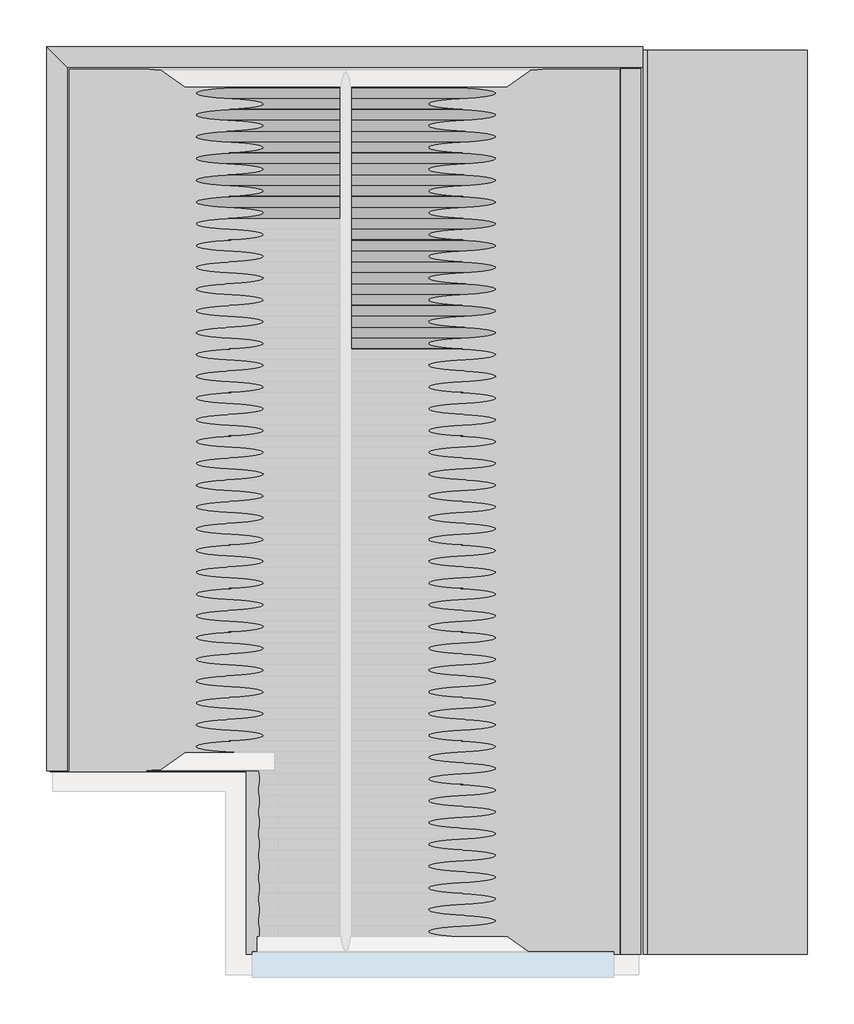
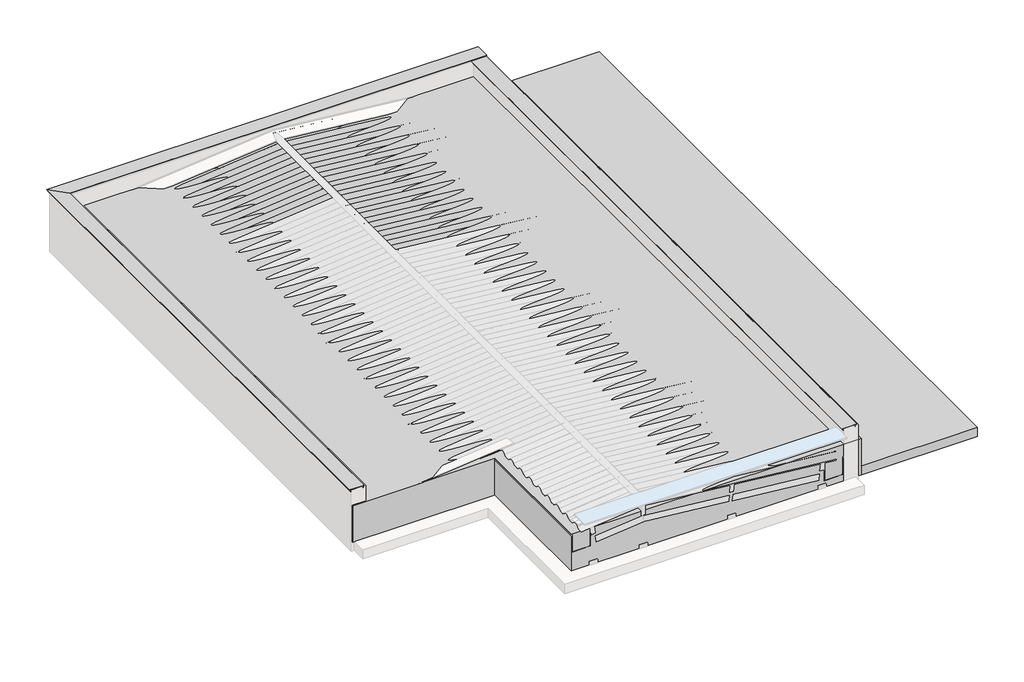
# One storey, part 4 of 4: 27 beams, 12 columns, 3 proxies.
"""IFC4 building model written with IfcOpenShell, lengths in millimetres."""

import ifcopenshell
import ifcopenshell.guid

model = None  # the IFC model being written
_history = None  # IfcOwnerHistory: only IFC2X3 demands one
_inside = {}  # id of a spatial element -> (the spatial element, [elements in it])
_under = {}  # id of a project, library or spatial element -> (it, [spatial elements below it])
_declared = {}  # id of a project -> (the project, [libraries it declares])
_typed = {}  # id of a type object -> (the type object, [elements of that type])
_made_of = {}  # id of a material, layer set ... -> (it, [elements and type objects made of it])


def new_model(schema):
    """Start an empty IFC model of exactly this schema.

    Asked for "IFC4X3", IfcOpenShell would pick the latest addendum, in which some entities
    have other attributes; the version numbers below select the first issue.
    IFC2X3 requires an IfcOwnerHistory on every rooted entity: one is made here for all.
    """
    global model, _history
    if schema == "IFC4X3":
        model = ifcopenshell.file(schema_version=(4, 3, 0, 0))
    else:
        model = ifcopenshell.file(schema=schema)
    _inside.clear()
    _under.clear()
    _declared.clear()
    _typed.clear()
    _made_of.clear()
    _history = None
    if model.schema == "IFC2X3":
        org = make("IfcOrganization", Name="unknown")
        user = make(
            "IfcPersonAndOrganization",
            ThePerson=make("IfcPerson", FamilyName="unknown"),
            TheOrganization=org,
        )
        app = make(
            "IfcApplication",
            ApplicationDeveloper=org,
            Version="unknown",
            ApplicationFullName="unknown",
            ApplicationIdentifier="unknown",
        )
        _history = make(
            "IfcOwnerHistory",
            OwningUser=user,
            OwningApplication=app,
            ChangeAction="ADDED",
            CreationDate=0,
        )
    return model


def make(cls, **values):
    """One entity of the class cls with the attributes given. An attribute that is None is left unset."""
    return model.create_entity(
        cls, **{name: value for name, value in values.items() if value is not None}
    )


def rooted(cls, **values):
    """An entity with a GlobalId (a new one), such as an element, a storey or a relation."""
    return make(cls, GlobalId=ifcopenshell.guid.new(), OwnerHistory=_history, **values)


def si_unit(unit_type, name, prefix=None):
    """IfcSIUnit, for example si_unit("LENGTHUNIT", "METRE", prefix="MILLI")."""
    return make("IfcSIUnit", UnitType=unit_type, Prefix=prefix, Name=name)


def assignment(units):
    """IfcUnitAssignment: the units of a project."""
    return None if units is None else make("IfcUnitAssignment", Units=units)


def point(xyz):
    """IfcCartesianPoint."""
    return None if xyz is None else make("IfcCartesianPoint", Coordinates=xyz)


def direction(xyz):
    """IfcDirection."""
    return None if xyz is None else make("IfcDirection", DirectionRatios=xyz)


def frame(location, z_axis=None, x_axis=None):
    """IfcAxis2Placement3D, a coordinate frame: its origin and axes. An axis left out is left unset."""
    return make(
        "IfcAxis2Placement3D",
        Location=point(location),
        Axis=direction(z_axis),
        RefDirection=direction(x_axis),
    )


def frame_2d(location, x_axis=None):
    """IfcAxis2Placement2D, a coordinate frame in the plane: its origin and x axis."""
    return make(
        "IfcAxis2Placement2D", Location=point(location), RefDirection=direction(x_axis)
    )


def origin():
    """The frame at (0, 0, 0) with its axes left unset."""
    return frame((0.0, 0.0, 0.0))


def place(relative_to, where):
    """IfcLocalPlacement: puts the frame where relative to a parent placement (None: the world)."""
    return make(
        "IfcLocalPlacement", PlacementRelTo=relative_to, RelativePlacement=where
    )


def context(
    kind, dimensions, precision=None, world=None, true_north=None, identifier=None
):
    """IfcGeometricRepresentationContext, for example the 3D "Model" context."""
    return make(
        "IfcGeometricRepresentationContext",
        ContextIdentifier=identifier,
        ContextType=kind,
        CoordinateSpaceDimension=dimensions,
        Precision=precision,
        WorldCoordinateSystem=world,
        TrueNorth=true_north,
    )


def project(units=None, contexts=None):
    """IfcProject with its units and contexts."""
    return rooted(
        "IfcProject",
        Name="project",
        RepresentationContexts=contexts,
        UnitsInContext=assignment(units),
    )


def spatial(cls, under=None, at=None, **own):
    """A site, building, storey or space (cls), placed at a placement, below another one or the project."""
    s = rooted(cls, ObjectPlacement=at, **own)
    if under is not None:
        _under.setdefault(under.id(), (under, []))[1].append(s)
    return s


def polyline(points):
    """IfcPolyline through the points."""
    return make("IfcPolyline", Points=[point(p) for p in points])


def circle_curve(where, radius):
    """IfcCircle in the frame where."""
    return make("IfcCircle", Position=where, Radius=radius)


def trimmed(basis, trim1, trim2, sense, master):
    """IfcTrimmedCurve: the piece of a basis curve between two trims."""
    return make(
        "IfcTrimmedCurve",
        BasisCurve=basis,
        Trim1=trim1,
        Trim2=trim2,
        SenseAgreement=sense,
        MasterRepresentation=master,
    )


def segment(curve, same_sense, transition):
    """IfcCompositeCurveSegment."""
    return make(
        "IfcCompositeCurveSegment",
        Transition=transition,
        SameSense=same_sense,
        ParentCurve=curve,
    )


def composite_curve(segments, self_intersect=None):
    """IfcCompositeCurve: segments joined end to end."""
    return make("IfcCompositeCurve", Segments=segments, SelfIntersect=self_intersect)


def outline(outer, holes=None, kind="AREA"):
    """IfcArbitraryClosedProfileDef: a profile drawn as a closed curve; with holes, ...WithVoids."""
    if holes is None:
        return make("IfcArbitraryClosedProfileDef", ProfileType=kind, OuterCurve=outer)
    return make(
        "IfcArbitraryProfileDefWithVoids",
        ProfileType=kind,
        OuterCurve=outer,
        InnerCurves=holes,
    )


def extrude(swept, where, along, depth):
    """IfcExtrudedAreaSolid: the profile swept, set in the frame where, extruded along a direction by depth."""
    return make(
        "IfcExtrudedAreaSolid",
        SweptArea=swept,
        Position=where,
        ExtrudedDirection=direction(along),
        Depth=depth,
    )


def faces_of(points, faces, orient=None, outer=None):
    """IfcFace entities. A face is a list of loops; a loop is a list of indices into points, from 0.

    orient and outer hold one flag for each loop. By default every Orientation is true, the
    first loop of a face is its IfcFaceOuterBound and the others are IfcFaceBound.
    """
    made = []
    for i, loops in enumerate(faces):
        bounds = []
        for j, loop in enumerate(loops):
            is_outer = j == 0 if outer is None else outer[i][j]
            bounds.append(
                make(
                    "IfcFaceOuterBound" if is_outer else "IfcFaceBound",
                    Bound=make("IfcPolyLoop", Polygon=[points[k] for k in loop]),
                    Orientation=True if orient is None else orient[i][j],
                )
            )
        made.append(make("IfcFace", Bounds=bounds))
    return made


def faceted_brep(points, faces, orient=None, outer=None, voids=None):
    """IfcFacetedBrep: a solid bounded by flat faces; with voids (closed shells), ...WithVoids."""
    shared = [point(p) for p in points]
    hull = make("IfcClosedShell", CfsFaces=faces_of(shared, faces, orient, outer))
    if voids is None:
        return make("IfcFacetedBrep", Outer=hull)
    return make(
        "IfcFacetedBrepWithVoids",
        Outer=hull,
        Voids=[
            make(cls, CfsFaces=faces_of(shared, fs, o, b)) for cls, fs, o, b in voids
        ],
    )


def shape(context_of_items, identifier, shape_type, items):
    """IfcShapeRepresentation: the items that make up one representation, for example the "Body"."""
    return make(
        "IfcShapeRepresentation",
        ContextOfItems=context_of_items,
        RepresentationIdentifier=identifier,
        RepresentationType=shape_type,
        Items=items,
    )


def source(mapping_origin, context_of_items, identifier, shape_type, items):
    """IfcRepresentationMap: a shape defined once, which mapped items show again and again."""
    return make(
        "IfcRepresentationMap",
        MappingOrigin=mapping_origin,
        MappedRepresentation=shape(context_of_items, identifier, shape_type, items),
    )


def transform(
    local_origin,
    x_axis=None,
    y_axis=None,
    z_axis=None,
    scale=None,
    scale2=None,
    scale3=None,
    uniform=True,
):
    """IfcCartesianTransformationOperator3D, or its non-uniform kind. x_axis, y_axis, z_axis: its Axis1, 2, 3."""
    if uniform:
        return make(
            "IfcCartesianTransformationOperator3D",
            Axis1=direction(x_axis),
            Axis2=direction(y_axis),
            LocalOrigin=point(local_origin),
            Scale=scale,
            Axis3=direction(z_axis),
        )
    return make(
        "IfcCartesianTransformationOperator3DnonUniform",
        Axis1=direction(x_axis),
        Axis2=direction(y_axis),
        LocalOrigin=point(local_origin),
        Scale=scale,
        Axis3=direction(z_axis),
        Scale2=scale2,
        Scale3=scale3,
    )


def mapped(mapping_source, mapping_target):
    """IfcMappedItem: shows the shape of a source again, moved by a transform."""
    return make(
        "IfcMappedItem", MappingSource=mapping_source, MappingTarget=mapping_target
    )


def made_of(thing, what):
    """Note that an element or type object is made of a material, layer set ...; save() writes the relation."""
    if what is not None:
        _made_of.setdefault(what.id(), (what, []))[1].append(thing)
    return thing


def element(
    cls,
    number,
    at=None,
    inside=None,
    cuts=None,
    type_object=None,
    material=None,
    context=None,
    identifier="Body",
    shape_type=None,
    held_by="IfcProductDefinitionShape",
    body=None,
    shapes=None,
    **own,
):
    """One element of the class cls, such as IfcWall. Its Tag is "e" and its number.

    at: its placement. inside: the storey or other place that contains it. cuts: it is an
    opening in that element (IfcRelVoidsElement). A single representation is given by context,
    identifier, shape_type and body (its items); several are given by shapes. held_by: the class
    of the entity that holds the representations. save() writes the other relations.
    """
    e = rooted(cls, Tag="e%d" % number, ObjectPlacement=at, **own)
    if body is not None:
        shapes = [shape(context, identifier, shape_type, body)]
    if shapes is not None:
        e.Representation = make(held_by, Representations=shapes)
    if inside is not None:
        _inside.setdefault(inside.id(), (inside, []))[1].append(e)
    if cuts is not None:
        rooted(
            "IfcRelVoidsElement", RelatingBuildingElement=cuts, RelatedOpeningElement=e
        )
    if type_object is not None:
        _typed.setdefault(type_object.id(), (type_object, []))[1].append(e)
    return made_of(e, material)


def aggregate(whole, parts):
    """IfcRelAggregates: a whole, such as a stair, and the parts it consists of."""
    return rooted("IfcRelAggregates", RelatingObject=whole, RelatedObjects=parts)


def save(model, path):
    """Write the relations noted so far, then the file.

    IfcRelAggregates (storeys below a building ...), IfcRelContainedInSpatialStructure (elements
    in a storey), IfcRelDefinesByType, IfcRelAssociatesMaterial and IfcRelDeclares: one each for
    every whole, place, type object, material and project.
    """
    for whole, parts in _under.values():
        aggregate(whole, parts)
    for where, things in _inside.values():
        rooted(
            "IfcRelContainedInSpatialStructure",
            RelatedElements=things,
            RelatingStructure=where,
        )
    for kind, things in _typed.values():
        rooted("IfcRelDefinesByType", RelatedObjects=things, RelatingType=kind)
    for what, things in _made_of.values():
        rooted("IfcRelAssociatesMaterial", RelatedObjects=things, RelatingMaterial=what)
    for by, libraries in _declared.values():
        rooted("IfcRelDeclares", RelatingContext=by, RelatedDefinitions=libraries)
    model.write(path)


def column_7d6827b5(model_context):
    return source(origin(), model_context, "Body", "SweptSolid", [
        extrude(outline(polyline([(30.0, 80.0), (30.0, -80.0), (-30.0, -80.0), (-30.0, 80.0), (30.0, 80.0)])), frame((0.0, 0.0, 4460.0), z_axis=(0.0, 0.0, 1.0), x_axis=(1.0, 0.0, 0.0)), (0.0, 0.0, 1.0), 466.0),
    ])


def column_c7348c99(model_context):
    return source(origin(), model_context, "Body", "SweptSolid", [
        extrude(outline(polyline([(30.0, 80.0), (30.0, -80.0), (-30.0, -80.0), (-30.0, 80.0), (30.0, 80.0)])), frame((0.0, 0.0, 4460.0), z_axis=(0.0, 0.0, 1.0), x_axis=(1.0, 0.0, 0.0)), (0.0, 0.0, 1.0), 372.8),
    ])


def column_6cc9e01b(model_context):
    return source(origin(), model_context, "Body", "SweptSolid", [
        extrude(outline(polyline([(30.0, 80.0), (30.0, -80.0), (-30.0, -80.0), (-30.0, 80.0), (30.0, 80.0)])), frame((0.0, 0.0, 4460.0), z_axis=(0.0, 0.0, 1.0), x_axis=(1.0, 0.0, 0.0)), (0.0, 0.0, 1.0), 233.0),
    ])


model = new_model("IFC4")

# Units and contexts
model_context = context("Model", 3, world=origin())
ifc_project = project(units=[si_unit("LENGTHUNIT", "METRE", prefix="MILLI")], contexts=[model_context])

# Site, building, storey
site = spatial("IfcSite", under=ifc_project)
building = spatial("IfcBuilding", under=site)
storey = spatial("IfcBuildingStorey", under=building, Name="COB. SALA ESTAR", Elevation=4400.0)

# Beams
placement = place(None, origin())
element("IfcBeam", 1, ObjectType="Madeira de lei : Berço 6x12cm", at=placement, inside=storey, context=model_context, shape_type="SweptSolid", body=[
    extrude(outline(polyline([(-3400.8557491, 5593.4722664), (-3280.8557491, 5593.4722664), (-3280.8557491, 4180.4300153), (-3400.8557491, 4180.4300153), (-3400.8557491, 5593.4722664)])), frame((0.0, 0.0, 4400.0), z_axis=(0.0, 0.0, 1.0), x_axis=(1.0, 0.0, 0.0)), (0.0, 0.0, 1.0), 60.0),
])
element("IfcBeam", 2, ObjectType="Madeira de lei : Berço 6x12cm", at=placement, inside=storey, context=model_context, shape_type="SweptSolid", body=[
    extrude(outline(polyline([(-2032.3324227, 4180.4300153), (-1912.3324227, 4180.4300153), (-1912.3324227, 2180.4300159), (-2032.3324227, 2180.4300159), (-2032.3324227, 4180.4300153)])), frame((0.0, 0.0, 4400.0), z_axis=(0.0, 0.0, 1.0), x_axis=(1.0, 0.0, 0.0)), (0.0, 0.0, 1.0), 60.0),
])
element("IfcBeam", 3, ObjectType="Madeira de lei : Berço 6x12cm", at=placement, inside=storey, context=model_context, shape_type="SweptSolid", body=[
    extrude(outline(polyline([(-2032.3324227, 5593.4722664), (-1912.3324227, 5593.4722664), (-1912.3324227, 4180.4300153), (-2032.3324227, 4180.4300153), (-2032.3324227, 5593.4722664)])), frame((0.0, 0.0, 4400.0), z_axis=(0.0, 0.0, 1.0), x_axis=(1.0, 0.0, 0.0)), (0.0, 0.0, 1.0), 60.0),
])
element("IfcBeam", 4, ObjectType="Madeira de lei : Berço 6x12cm", at=placement, inside=storey, context=model_context, shape_type="SweptSolid", body=[
    extrude(outline(polyline([(-634.0324227, 4180.4300153), (-514.0324227, 4180.4300153), (-514.0324227, 2180.4300159), (-634.0324227, 2180.4300159), (-634.0324227, 4180.4300153)])), frame((0.0, 0.0, 4400.0), z_axis=(0.0, 0.0, 1.0), x_axis=(1.0, 0.0, 0.0)), (0.0, 0.0, 1.0), 60.0),
])
element("IfcBeam", 5, ObjectType="Madeira de lei : Berço 6x12cm", at=placement, inside=storey, context=model_context, shape_type="SweptSolid", body=[
    extrude(outline(polyline([(-634.0324227, 5593.4722664), (-514.0324227, 5593.4722664), (-514.0324227, 4180.4300153), (-634.0324227, 4180.4300153), (-634.0324227, 5593.4722664)])), frame((0.0, 0.0, 4400.0), z_axis=(0.0, 0.0, 1.0), x_axis=(1.0, 0.0, 0.0)), (0.0, 0.0, 1.0), 60.0),
])
element("IfcBeam", 6, ObjectType="Madeira de lei : Berço 6x12cm", at=placement, inside=storey, context=model_context, shape_type="SweptSolid", body=[
    extrude(outline(polyline([(-6167.5301913, 5593.4722664), (-6047.5301913, 5593.4722664), (-6047.5301913, 4180.4300153), (-6167.5301913, 4180.4300153), (-6167.5301913, 5593.4722664)])), frame((0.0, 0.0, 4400.0), z_axis=(0.0, 0.0, 1.0), x_axis=(1.0, 0.0, 0.0)), (0.0, 0.0, 1.0), 60.0),
])
element("IfcBeam", 7, ObjectType="Madeira de lei : Berço 6x12cm", at=placement, inside=storey, context=model_context, shape_type="SweptSolid", body=[
    extrude(outline(polyline([(-4769.2301913, 5593.4722664), (-4649.2301913, 5593.4722664), (-4649.2301913, 4180.4300153), (-4769.2301913, 4180.4300153), (-4769.2301913, 5593.4722664)])), frame((0.0, 0.0, 4400.0), z_axis=(0.0, 0.0, 1.0), x_axis=(1.0, 0.0, 0.0)), (0.0, 0.0, 1.0), 60.0),
])
element("IfcBeam", 8, ObjectType="Telha Ondulada : Fibrocimento", at=placement, inside=storey, context=model_context, shape_type="SweptSolid", body=[
    extrude(outline(composite_curve([segment(trimmed(circle_curve(frame_2d((-58.7002978, -53.2060538)), 66.7939461), [point((-29.3501489, 6.7939462))], [point((-29.3501489, -113.2060538))], False, "CARTESIAN"), True, "CONTINUOUS"), segment(polyline([(-29.3501489, -113.2060538), (-31.5472154, -108.7146288)]), True, "CONTINUOUS"), segment(trimmed(circle_curve(frame_2d((-58.7002978, -53.2060538)), 61.7939461), [point((-31.5472154, -108.7146288))], [point((-31.5472154, 2.3025211))], True, "CARTESIAN"), True, "CONTINUOUS"), segment(trimmed(circle_curve(frame_2d((0.0, 66.7939462)), 71.7939461), [point((-31.5472154, 2.3025211))], [point((-31.5472154, 131.2853712))], False, "CARTESIAN"), True, "CONTINUOUS"), segment(polyline([(-31.5472154, 131.2853712), (-29.3501489, 126.7939462)]), True, "CONTINUOUS"), segment(trimmed(circle_curve(frame_2d((0.0, 66.7939462)), 66.7939461), [point((-29.3501489, 126.7939462))], [point((-29.3501489, 6.7939462))], True, "CARTESIAN"), True, "CONTINUOUS")], self_intersect=False)), frame((-6307.6707245, 4045.326948, 4862.7215886), z_axis=(0.9950371902099892, 0.0, 0.09950371902099954), x_axis=(-0.09950371902099954, 0.0, 0.9950371902099892)), (0.0, 0.0, 1.0), 2972.5075682),
])
element("IfcBeam", 9, ObjectType="Telha Ondulada : Fibrocimento", at=placement, inside=storey, context=model_context, shape_type="SweptSolid", body=[
    extrude(outline(composite_curve([segment(trimmed(circle_curve(frame_2d((-58.7002978, -53.2060538)), 66.7939461), [point((-29.3501489, 6.7939462))], [point((-29.3501489, -113.2060538))], False, "CARTESIAN"), True, "CONTINUOUS"), segment(polyline([(-29.3501489, -113.2060538), (-31.5472154, -108.7146288)]), True, "CONTINUOUS"), segment(trimmed(circle_curve(frame_2d((-58.7002978, -53.2060538)), 61.7939461), [point((-31.5472154, -108.7146288))], [point((-31.5472154, 2.3025211))], True, "CARTESIAN"), True, "CONTINUOUS"), segment(trimmed(circle_curve(frame_2d((0.0, 66.7939462)), 71.7939461), [point((-31.5472154, 2.3025211))], [point((-31.5472154, 131.2853712))], False, "CARTESIAN"), True, "CONTINUOUS"), segment(polyline([(-31.5472154, 131.2853712), (-29.3501489, 126.7939462)]), True, "CONTINUOUS"), segment(trimmed(circle_curve(frame_2d((0.0, 66.7939462)), 66.7939461), [point((-29.3501489, 126.7939462))], [point((-29.3501489, 6.7939462))], True, "CARTESIAN"), True, "CONTINUOUS")], self_intersect=False)), frame((-6307.6707245, 4289.826948, 4862.7215886), z_axis=(0.9950371902099892, 0.0, 0.09950371902099969), x_axis=(-0.09950371902099969, 0.0, 0.9950371902099892)), (0.0, 0.0, 1.0), 2972.5075682),
])
element("IfcBeam", 10, ObjectType="Telha Ondulada : Fibrocimento", at=placement, inside=storey, context=model_context, shape_type="SweptSolid", body=[
    extrude(outline(composite_curve([segment(trimmed(circle_curve(frame_2d((-58.7002978, -53.2060538)), 66.7939461), [point((-29.3501489, 6.7939462))], [point((-29.3501489, -113.2060538))], False, "CARTESIAN"), True, "CONTINUOUS"), segment(polyline([(-29.3501489, -113.2060538), (-31.5472154, -108.7146288)]), True, "CONTINUOUS"), segment(trimmed(circle_curve(frame_2d((-58.7002978, -53.2060538)), 61.7939461), [point((-31.5472154, -108.7146288))], [point((-31.5472154, 2.3025211))], True, "CARTESIAN"), True, "CONTINUOUS"), segment(trimmed(circle_curve(frame_2d((0.0, 66.7939462)), 71.7939461), [point((-31.5472154, 2.3025211))], [point((-31.5472154, 131.2853712))], False, "CARTESIAN"), True, "CONTINUOUS"), segment(polyline([(-31.5472154, 131.2853712), (-29.3501489, 126.7939462)]), True, "CONTINUOUS"), segment(trimmed(circle_curve(frame_2d((0.0, 66.7939462)), 66.7939461), [point((-29.3501489, 126.7939462))], [point((-29.3501489, 6.7939462))], True, "CARTESIAN"), True, "CONTINUOUS")], self_intersect=False)), frame((-6307.6707245, 4534.326948, 4862.7215886), z_axis=(0.9950371902099892, 0.0, 0.09950371902099972), x_axis=(-0.09950371902099972, 0.0, 0.9950371902099892)), (0.0, 0.0, 1.0), 2972.5075682),
])
element("IfcBeam", 11, ObjectType="Telha Ondulada : Fibrocimento", at=placement, inside=storey, context=model_context, shape_type="SweptSolid", body=[
    extrude(outline(composite_curve([segment(trimmed(circle_curve(frame_2d((-58.7002978, -53.2060538)), 66.7939461), [point((-29.3501489, 6.7939462))], [point((-29.3501489, -113.2060538))], False, "CARTESIAN"), True, "CONTINUOUS"), segment(polyline([(-29.3501489, -113.2060538), (-31.5472154, -108.7146288)]), True, "CONTINUOUS"), segment(trimmed(circle_curve(frame_2d((-58.7002978, -53.2060538)), 61.7939461), [point((-31.5472154, -108.7146288))], [point((-31.5472154, 2.3025211))], True, "CARTESIAN"), True, "CONTINUOUS"), segment(trimmed(circle_curve(frame_2d((0.0, 66.7939462)), 71.7939461), [point((-31.5472154, 2.3025211))], [point((-31.5472154, 131.2853712))], False, "CARTESIAN"), True, "CONTINUOUS"), segment(polyline([(-31.5472154, 131.2853712), (-29.3501489, 126.7939462)]), True, "CONTINUOUS"), segment(trimmed(circle_curve(frame_2d((0.0, 66.7939462)), 66.7939461), [point((-29.3501489, 126.7939462))], [point((-29.3501489, 6.7939462))], True, "CARTESIAN"), True, "CONTINUOUS")], self_intersect=False)), frame((-6307.6707245, 4778.826948, 4862.7215886), z_axis=(0.9950371902099892, 0.0, 0.09950371902099972), x_axis=(-0.09950371902099972, 0.0, 0.9950371902099892)), (0.0, 0.0, 1.0), 2972.5075682),
])
element("IfcBeam", 12, ObjectType="Telha Ondulada : Fibrocimento", at=placement, inside=storey, context=model_context, shape_type="SweptSolid", body=[
    extrude(outline(composite_curve([segment(trimmed(circle_curve(frame_2d((-58.7002978, -53.2060538)), 66.7939461), [point((-29.3501489, 6.7939462))], [point((-29.3501489, -113.2060538))], False, "CARTESIAN"), True, "CONTINUOUS"), segment(polyline([(-29.3501489, -113.2060538), (-31.5472154, -108.7146288)]), True, "CONTINUOUS"), segment(trimmed(circle_curve(frame_2d((-58.7002978, -53.2060538)), 61.7939461), [point((-31.5472154, -108.7146288))], [point((-31.5472154, 2.3025211))], True, "CARTESIAN"), True, "CONTINUOUS"), segment(trimmed(circle_curve(frame_2d((0.0, 66.7939462)), 71.7939461), [point((-31.5472154, 2.3025211))], [point((-31.5472154, 131.2853712))], False, "CARTESIAN"), True, "CONTINUOUS"), segment(polyline([(-31.5472154, 131.2853712), (-29.3501489, 126.7939462)]), True, "CONTINUOUS"), segment(trimmed(circle_curve(frame_2d((0.0, 66.7939462)), 66.7939461), [point((-29.3501489, 126.7939462))], [point((-29.3501489, 6.7939462))], True, "CARTESIAN"), True, "CONTINUOUS")], self_intersect=False)), frame((-6307.6707245, 5023.326948, 4862.7215886), z_axis=(0.9950371902099892, 0.0, 0.09950371902099968), x_axis=(-0.09950371902099968, 0.0, 0.9950371902099892)), (0.0, 0.0, 1.0), 2972.5075682),
])
element("IfcBeam", 13, ObjectType="Telha Ondulada : Fibrocimento", at=placement, inside=storey, context=model_context, shape_type="SweptSolid", body=[
    extrude(outline(composite_curve([segment(trimmed(circle_curve(frame_2d((-58.7002978, -53.2060538)), 66.7939461), [point((-29.3501489, 6.7939462))], [point((-29.3501489, -113.2060538))], False, "CARTESIAN"), True, "CONTINUOUS"), segment(polyline([(-29.3501489, -113.2060538), (-31.5472154, -108.7146288)]), True, "CONTINUOUS"), segment(trimmed(circle_curve(frame_2d((-58.7002978, -53.2060538)), 61.7939461), [point((-31.5472154, -108.7146288))], [point((-31.5472154, 2.3025211))], True, "CARTESIAN"), True, "CONTINUOUS"), segment(trimmed(circle_curve(frame_2d((0.0, 66.7939462)), 71.7939461), [point((-31.5472154, 2.3025211))], [point((-31.5472154, 131.2853712))], False, "CARTESIAN"), True, "CONTINUOUS"), segment(polyline([(-31.5472154, 131.2853712), (-29.3501489, 126.7939462)]), True, "CONTINUOUS"), segment(trimmed(circle_curve(frame_2d((0.0, 66.7939462)), 66.7939461), [point((-29.3501489, 126.7939462))], [point((-29.3501489, 6.7939462))], True, "CARTESIAN"), True, "CONTINUOUS")], self_intersect=False)), frame((-6307.6707245, 5267.826948, 4862.7215886), z_axis=(0.9950371902099892, 0.0, 0.09950371902099968), x_axis=(-0.09950371902099968, 0.0, 0.9950371902099892)), (0.0, 0.0, 1.0), 2972.5075682),
])
element("IfcBeam", 14, ObjectType="Telha Ondulada : Fibrocimento", at=placement, inside=storey, context=model_context, shape_type="SweptSolid", body=[
    extrude(outline(composite_curve([segment(trimmed(circle_curve(frame_2d((-58.7002978, -53.2060538)), 66.7939461), [point((-29.3501489, 6.7939462))], [point((-29.3501489, -113.2060538))], False, "CARTESIAN"), True, "CONTINUOUS"), segment(polyline([(-29.3501489, -113.2060538), (-31.5472154, -108.7146288)]), True, "CONTINUOUS"), segment(trimmed(circle_curve(frame_2d((-58.7002978, -53.2060538)), 61.7939461), [point((-31.5472154, -108.7146288))], [point((-31.5472154, 2.3025211))], True, "CARTESIAN"), True, "CONTINUOUS"), segment(trimmed(circle_curve(frame_2d((0.0, 66.7939462)), 71.7939461), [point((-31.5472154, 2.3025211))], [point((-31.5472154, 131.2853712))], False, "CARTESIAN"), True, "CONTINUOUS"), segment(polyline([(-31.5472154, 131.2853712), (-29.3501489, 126.7939462)]), True, "CONTINUOUS"), segment(trimmed(circle_curve(frame_2d((0.0, 66.7939462)), 66.7939461), [point((-29.3501489, 126.7939462))], [point((-29.3501489, 6.7939462))], True, "CARTESIAN"), True, "CONTINUOUS")], self_intersect=False)), frame((-6307.6707245, 5512.326948, 4862.7215886), z_axis=(0.9950371902099892, 0.0, 0.09950371902099951), x_axis=(-0.09950371902099951, 0.0, 0.9950371902099892)), (0.0, 0.0, 1.0), 2972.5075682),
])
element("IfcBeam", 15, ObjectType="Telha Ondulada : Fibrocimento", at=placement, inside=storey, context=model_context, shape_type="SweptSolid", body=[
    extrude(outline(composite_curve([segment(trimmed(circle_curve(frame_2d((0.0, 66.7939462)), 66.7939461), [point((29.3501489, 6.7939462))], [point((29.3501489, 126.7939462))], True, "CARTESIAN"), True, "CONTINUOUS"), segment(polyline([(29.3501489, 126.7939462), (31.5472154, 131.2853712)]), True, "CONTINUOUS"), segment(trimmed(circle_curve(frame_2d((0.0, 66.7939462)), 71.7939461), [point((31.5472154, 131.2853712))], [point((31.5472154, 2.3025211))], False, "CARTESIAN"), True, "CONTINUOUS"), segment(trimmed(circle_curve(frame_2d((58.7002978, -53.2060538)), 61.7939461), [point((31.5472154, 2.3025211))], [point((31.5472154, -108.7146288))], True, "CARTESIAN"), True, "CONTINUOUS"), segment(polyline([(31.5472154, -108.7146288), (29.3501489, -113.2060538)]), True, "CONTINUOUS"), segment(trimmed(circle_curve(frame_2d((58.7002978, -53.2060538)), 66.7939461), [point((29.3501489, -113.2060538))], [point((29.3501489, 6.7939462))], False, "CARTESIAN"), True, "CONTINUOUS")], self_intersect=False)), frame((-373.8918894, 2578.326948, 4862.7215886), z_axis=(-0.9950371902099892, 0.0, 0.09950371902099946), x_axis=(-0.09950371902099946, 0.0, -0.9950371902099892)), (0.0, 0.0, 1.0), 2972.5075682),
])
element("IfcBeam", 16, ObjectType="Telha Ondulada : Fibrocimento", at=placement, inside=storey, context=model_context, shape_type="SweptSolid", body=[
    extrude(outline(composite_curve([segment(trimmed(circle_curve(frame_2d((0.0, 66.7939462)), 66.7939461), [point((29.3501489, 6.7939462))], [point((29.3501489, 126.7939462))], True, "CARTESIAN"), True, "CONTINUOUS"), segment(polyline([(29.3501489, 126.7939462), (31.5472154, 131.2853712)]), True, "CONTINUOUS"), segment(trimmed(circle_curve(frame_2d((0.0, 66.7939462)), 71.7939461), [point((31.5472154, 131.2853712))], [point((31.5472154, 2.3025211))], False, "CARTESIAN"), True, "CONTINUOUS"), segment(trimmed(circle_curve(frame_2d((58.7002978, -53.2060538)), 61.7939461), [point((31.5472154, 2.3025211))], [point((31.5472154, -108.7146288))], True, "CARTESIAN"), True, "CONTINUOUS"), segment(polyline([(31.5472154, -108.7146288), (29.3501489, -113.2060538)]), True, "CONTINUOUS"), segment(trimmed(circle_curve(frame_2d((58.7002978, -53.2060538)), 66.7939461), [point((29.3501489, -113.2060538))], [point((29.3501489, 6.7939462))], False, "CARTESIAN"), True, "CONTINUOUS")], self_intersect=False)), frame((-373.8918894, 2822.826948, 4862.7215886), z_axis=(-0.9950371902099892, 0.0, 0.09950371902099946), x_axis=(-0.09950371902099946, 0.0, -0.9950371902099892)), (0.0, 0.0, 1.0), 2972.5075682),
])
element("IfcBeam", 17, ObjectType="Telha Ondulada : Fibrocimento", at=placement, inside=storey, context=model_context, shape_type="SweptSolid", body=[
    extrude(outline(composite_curve([segment(trimmed(circle_curve(frame_2d((0.0, 66.7939462)), 66.7939461), [point((29.3501489, 6.7939462))], [point((29.3501489, 126.7939462))], True, "CARTESIAN"), True, "CONTINUOUS"), segment(polyline([(29.3501489, 126.7939462), (31.5472154, 131.2853712)]), True, "CONTINUOUS"), segment(trimmed(circle_curve(frame_2d((0.0, 66.7939462)), 71.7939461), [point((31.5472154, 131.2853712))], [point((31.5472154, 2.3025211))], False, "CARTESIAN"), True, "CONTINUOUS"), segment(trimmed(circle_curve(frame_2d((58.7002978, -53.2060538)), 61.7939461), [point((31.5472154, 2.3025211))], [point((31.5472154, -108.7146288))], True, "CARTESIAN"), True, "CONTINUOUS"), segment(polyline([(31.5472154, -108.7146288), (29.3501489, -113.2060538)]), True, "CONTINUOUS"), segment(trimmed(circle_curve(frame_2d((58.7002978, -53.2060538)), 66.7939461), [point((29.3501489, -113.2060538))], [point((29.3501489, 6.7939462))], False, "CARTESIAN"), True, "CONTINUOUS")], self_intersect=False)), frame((-373.8918894, 3067.326948, 4862.7215886), z_axis=(-0.9950371902099892, 0.0, 0.09950371902099946), x_axis=(-0.09950371902099946, 0.0, -0.9950371902099892)), (0.0, 0.0, 1.0), 2972.5075682),
])
element("IfcBeam", 18, ObjectType="Telha Ondulada : Fibrocimento", at=placement, inside=storey, context=model_context, shape_type="SweptSolid", body=[
    extrude(outline(composite_curve([segment(trimmed(circle_curve(frame_2d((0.0, 66.7939462)), 66.7939461), [point((29.3501489, 6.7939462))], [point((29.3501489, 126.7939462))], True, "CARTESIAN"), True, "CONTINUOUS"), segment(polyline([(29.3501489, 126.7939462), (31.5472154, 131.2853712)]), True, "CONTINUOUS"), segment(trimmed(circle_curve(frame_2d((0.0, 66.7939462)), 71.7939461), [point((31.5472154, 131.2853712))], [point((31.5472154, 2.3025211))], False, "CARTESIAN"), True, "CONTINUOUS"), segment(trimmed(circle_curve(frame_2d((58.7002978, -53.2060538)), 61.7939461), [point((31.5472154, 2.3025211))], [point((31.5472154, -108.7146288))], True, "CARTESIAN"), True, "CONTINUOUS"), segment(polyline([(31.5472154, -108.7146288), (29.3501489, -113.2060538)]), True, "CONTINUOUS"), segment(trimmed(circle_curve(frame_2d((58.7002978, -53.2060538)), 66.7939461), [point((29.3501489, -113.2060538))], [point((29.3501489, 6.7939462))], False, "CARTESIAN"), True, "CONTINUOUS")], self_intersect=False)), frame((-373.8918894, 3311.826948, 4862.7215886), z_axis=(-0.9950371902099892, 0.0, 0.09950371902099946), x_axis=(-0.09950371902099946, 0.0, -0.9950371902099892)), (0.0, 0.0, 1.0), 2972.5075682),
])
element("IfcBeam", 19, ObjectType="Telha Ondulada : Fibrocimento", at=placement, inside=storey, context=model_context, shape_type="SweptSolid", body=[
    extrude(outline(composite_curve([segment(trimmed(circle_curve(frame_2d((0.0, 66.7939462)), 66.7939461), [point((29.3501489, 6.7939462))], [point((29.3501489, 126.7939462))], True, "CARTESIAN"), True, "CONTINUOUS"), segment(polyline([(29.3501489, 126.7939462), (31.5472154, 131.2853712)]), True, "CONTINUOUS"), segment(trimmed(circle_curve(frame_2d((0.0, 66.7939462)), 71.7939461), [point((31.5472154, 131.2853712))], [point((31.5472154, 2.3025211))], False, "CARTESIAN"), True, "CONTINUOUS"), segment(trimmed(circle_curve(frame_2d((58.7002978, -53.2060538)), 61.7939461), [point((31.5472154, 2.3025211))], [point((31.5472154, -108.7146288))], True, "CARTESIAN"), True, "CONTINUOUS"), segment(polyline([(31.5472154, -108.7146288), (29.3501489, -113.2060538)]), True, "CONTINUOUS"), segment(trimmed(circle_curve(frame_2d((58.7002978, -53.2060538)), 66.7939461), [point((29.3501489, -113.2060538))], [point((29.3501489, 6.7939462))], False, "CARTESIAN"), True, "CONTINUOUS")], self_intersect=False)), frame((-373.8918894, 3556.326948, 4862.7215886), z_axis=(-0.9950371902099892, 0.0, 0.09950371902099946), x_axis=(-0.09950371902099946, 0.0, -0.9950371902099892)), (0.0, 0.0, 1.0), 2972.5075682),
])
element("IfcBeam", 20, ObjectType="Telha Ondulada : Fibrocimento", at=placement, inside=storey, context=model_context, shape_type="SweptSolid", body=[
    extrude(outline(composite_curve([segment(trimmed(circle_curve(frame_2d((0.0, 66.7939462)), 66.7939461), [point((29.3501489, 6.7939462))], [point((29.3501489, 126.7939462))], True, "CARTESIAN"), True, "CONTINUOUS"), segment(polyline([(29.3501489, 126.7939462), (31.5472154, 131.2853712)]), True, "CONTINUOUS"), segment(trimmed(circle_curve(frame_2d((0.0, 66.7939462)), 71.7939461), [point((31.5472154, 131.2853712))], [point((31.5472154, 2.3025211))], False, "CARTESIAN"), True, "CONTINUOUS"), segment(trimmed(circle_curve(frame_2d((58.7002978, -53.2060538)), 61.7939461), [point((31.5472154, 2.3025211))], [point((31.5472154, -108.7146288))], True, "CARTESIAN"), True, "CONTINUOUS"), segment(polyline([(31.5472154, -108.7146288), (29.3501489, -113.2060538)]), True, "CONTINUOUS"), segment(trimmed(circle_curve(frame_2d((58.7002978, -53.2060538)), 66.7939461), [point((29.3501489, -113.2060538))], [point((29.3501489, 6.7939462))], False, "CARTESIAN"), True, "CONTINUOUS")], self_intersect=False)), frame((-373.8918894, 3800.826948, 4862.7215886), z_axis=(-0.9950371902099892, 0.0, 0.09950371902099946), x_axis=(-0.09950371902099946, 0.0, -0.9950371902099892)), (0.0, 0.0, 1.0), 2972.5075682),
])
element("IfcBeam", 21, ObjectType="Telha Ondulada : Fibrocimento", at=placement, inside=storey, context=model_context, shape_type="SweptSolid", body=[
    extrude(outline(composite_curve([segment(trimmed(circle_curve(frame_2d((0.0, 66.7939462)), 66.7939461), [point((29.3501489, 6.7939462))], [point((29.3501489, 126.7939462))], True, "CARTESIAN"), True, "CONTINUOUS"), segment(polyline([(29.3501489, 126.7939462), (31.5472154, 131.2853712)]), True, "CONTINUOUS"), segment(trimmed(circle_curve(frame_2d((0.0, 66.7939462)), 71.7939461), [point((31.5472154, 131.2853712))], [point((31.5472154, 2.3025211))], False, "CARTESIAN"), True, "CONTINUOUS"), segment(trimmed(circle_curve(frame_2d((58.7002978, -53.2060538)), 61.7939461), [point((31.5472154, 2.3025211))], [point((31.5472154, -108.7146288))], True, "CARTESIAN"), True, "CONTINUOUS"), segment(polyline([(31.5472154, -108.7146288), (29.3501489, -113.2060538)]), True, "CONTINUOUS"), segment(trimmed(circle_curve(frame_2d((58.7002978, -53.2060538)), 66.7939461), [point((29.3501489, -113.2060538))], [point((29.3501489, 6.7939462))], False, "CARTESIAN"), True, "CONTINUOUS")], self_intersect=False)), frame((-373.8918894, 4045.326948, 4862.7215886), z_axis=(-0.9950371902099892, 0.0, 0.09950371902099946), x_axis=(-0.09950371902099946, 0.0, -0.9950371902099892)), (0.0, 0.0, 1.0), 2972.5075682),
])
element("IfcBeam", 22, ObjectType="Telha Ondulada : Fibrocimento", at=placement, inside=storey, context=model_context, shape_type="SweptSolid", body=[
    extrude(outline(composite_curve([segment(trimmed(circle_curve(frame_2d((0.0, 66.7939462)), 66.7939461), [point((29.3501489, 6.7939462))], [point((29.3501489, 126.7939462))], True, "CARTESIAN"), True, "CONTINUOUS"), segment(polyline([(29.3501489, 126.7939462), (31.5472154, 131.2853712)]), True, "CONTINUOUS"), segment(trimmed(circle_curve(frame_2d((0.0, 66.7939462)), 71.7939461), [point((31.5472154, 131.2853712))], [point((31.5472154, 2.3025211))], False, "CARTESIAN"), True, "CONTINUOUS"), segment(trimmed(circle_curve(frame_2d((58.7002978, -53.2060538)), 61.7939461), [point((31.5472154, 2.3025211))], [point((31.5472154, -108.7146288))], True, "CARTESIAN"), True, "CONTINUOUS"), segment(polyline([(31.5472154, -108.7146288), (29.3501489, -113.2060538)]), True, "CONTINUOUS"), segment(trimmed(circle_curve(frame_2d((58.7002978, -53.2060538)), 66.7939461), [point((29.3501489, -113.2060538))], [point((29.3501489, 6.7939462))], False, "CARTESIAN"), True, "CONTINUOUS")], self_intersect=False)), frame((-373.8918894, 4289.826948, 4862.7215886), z_axis=(-0.9950371902099892, 0.0, 0.09950371902099946), x_axis=(-0.09950371902099946, 0.0, -0.9950371902099892)), (0.0, 0.0, 1.0), 2972.5075682),
])
element("IfcBeam", 23, ObjectType="Telha Ondulada : Fibrocimento", at=placement, inside=storey, context=model_context, shape_type="SweptSolid", body=[
    extrude(outline(composite_curve([segment(trimmed(circle_curve(frame_2d((0.0, 66.7939462)), 66.7939461), [point((29.3501489, 6.7939462))], [point((29.3501489, 126.7939462))], True, "CARTESIAN"), True, "CONTINUOUS"), segment(polyline([(29.3501489, 126.7939462), (31.5472154, 131.2853712)]), True, "CONTINUOUS"), segment(trimmed(circle_curve(frame_2d((0.0, 66.7939462)), 71.7939461), [point((31.5472154, 131.2853712))], [point((31.5472154, 2.3025211))], False, "CARTESIAN"), True, "CONTINUOUS"), segment(trimmed(circle_curve(frame_2d((58.7002978, -53.2060538)), 61.7939461), [point((31.5472154, 2.3025211))], [point((31.5472154, -108.7146288))], True, "CARTESIAN"), True, "CONTINUOUS"), segment(polyline([(31.5472154, -108.7146288), (29.3501489, -113.2060538)]), True, "CONTINUOUS"), segment(trimmed(circle_curve(frame_2d((58.7002978, -53.2060538)), 66.7939461), [point((29.3501489, -113.2060538))], [point((29.3501489, 6.7939462))], False, "CARTESIAN"), True, "CONTINUOUS")], self_intersect=False)), frame((-373.8918894, 4534.326948, 4862.7215886), z_axis=(-0.9950371902099892, 0.0, 0.09950371902099946), x_axis=(-0.09950371902099946, 0.0, -0.9950371902099892)), (0.0, 0.0, 1.0), 2972.5075682),
])
element("IfcBeam", 24, ObjectType="Telha Ondulada : Fibrocimento", at=placement, inside=storey, context=model_context, shape_type="SweptSolid", body=[
    extrude(outline(composite_curve([segment(trimmed(circle_curve(frame_2d((0.0, 66.7939462)), 66.7939461), [point((29.3501489, 6.7939462))], [point((29.3501489, 126.7939462))], True, "CARTESIAN"), True, "CONTINUOUS"), segment(polyline([(29.3501489, 126.7939462), (31.5472154, 131.2853712)]), True, "CONTINUOUS"), segment(trimmed(circle_curve(frame_2d((0.0, 66.7939462)), 71.7939461), [point((31.5472154, 131.2853712))], [point((31.5472154, 2.3025211))], False, "CARTESIAN"), True, "CONTINUOUS"), segment(trimmed(circle_curve(frame_2d((58.7002978, -53.2060538)), 61.7939461), [point((31.5472154, 2.3025211))], [point((31.5472154, -108.7146288))], True, "CARTESIAN"), True, "CONTINUOUS"), segment(polyline([(31.5472154, -108.7146288), (29.3501489, -113.2060538)]), True, "CONTINUOUS"), segment(trimmed(circle_curve(frame_2d((58.7002978, -53.2060538)), 66.7939461), [point((29.3501489, -113.2060538))], [point((29.3501489, 6.7939462))], False, "CARTESIAN"), True, "CONTINUOUS")], self_intersect=False)), frame((-373.8918894, 4778.826948, 4862.7215886), z_axis=(-0.9950371902099892, 0.0, 0.09950371902099946), x_axis=(-0.09950371902099946, 0.0, -0.9950371902099892)), (0.0, 0.0, 1.0), 2972.5075682),
])
element("IfcBeam", 25, ObjectType="Telha Ondulada : Fibrocimento", at=placement, inside=storey, context=model_context, shape_type="SweptSolid", body=[
    extrude(outline(composite_curve([segment(trimmed(circle_curve(frame_2d((0.0, 66.7939462)), 66.7939461), [point((29.3501489, 6.7939462))], [point((29.3501489, 126.7939462))], True, "CARTESIAN"), True, "CONTINUOUS"), segment(polyline([(29.3501489, 126.7939462), (31.5472154, 131.2853712)]), True, "CONTINUOUS"), segment(trimmed(circle_curve(frame_2d((0.0, 66.7939462)), 71.7939461), [point((31.5472154, 131.2853712))], [point((31.5472154, 2.3025211))], False, "CARTESIAN"), True, "CONTINUOUS"), segment(trimmed(circle_curve(frame_2d((58.7002978, -53.2060538)), 61.7939461), [point((31.5472154, 2.3025211))], [point((31.5472154, -108.7146288))], True, "CARTESIAN"), True, "CONTINUOUS"), segment(polyline([(31.5472154, -108.7146288), (29.3501489, -113.2060538)]), True, "CONTINUOUS"), segment(trimmed(circle_curve(frame_2d((58.7002978, -53.2060538)), 66.7939461), [point((29.3501489, -113.2060538))], [point((29.3501489, 6.7939462))], False, "CARTESIAN"), True, "CONTINUOUS")], self_intersect=False)), frame((-373.8918894, 5023.326948, 4862.7215886), z_axis=(-0.9950371902099892, 0.0, 0.09950371902099946), x_axis=(-0.09950371902099946, 0.0, -0.9950371902099892)), (0.0, 0.0, 1.0), 2972.5075682),
])
element("IfcBeam", 26, ObjectType="Telha Ondulada : Fibrocimento", at=placement, inside=storey, context=model_context, shape_type="SweptSolid", body=[
    extrude(outline(composite_curve([segment(trimmed(circle_curve(frame_2d((0.0, 66.7939462)), 66.7939461), [point((29.3501489, 6.7939462))], [point((29.3501489, 126.7939462))], True, "CARTESIAN"), True, "CONTINUOUS"), segment(polyline([(29.3501489, 126.7939462), (31.5472154, 131.2853712)]), True, "CONTINUOUS"), segment(trimmed(circle_curve(frame_2d((0.0, 66.7939462)), 71.7939461), [point((31.5472154, 131.2853712))], [point((31.5472154, 2.3025211))], False, "CARTESIAN"), True, "CONTINUOUS"), segment(trimmed(circle_curve(frame_2d((58.7002978, -53.2060538)), 61.7939461), [point((31.5472154, 2.3025211))], [point((31.5472154, -108.7146288))], True, "CARTESIAN"), True, "CONTINUOUS"), segment(polyline([(31.5472154, -108.7146288), (29.3501489, -113.2060538)]), True, "CONTINUOUS"), segment(trimmed(circle_curve(frame_2d((58.7002978, -53.2060538)), 66.7939461), [point((29.3501489, -113.2060538))], [point((29.3501489, 6.7939462))], False, "CARTESIAN"), True, "CONTINUOUS")], self_intersect=False)), frame((-373.8918894, 5267.826948, 4862.7215886), z_axis=(-0.9950371902099892, 0.0, 0.09950371902099946), x_axis=(-0.09950371902099946, 0.0, -0.9950371902099892)), (0.0, 0.0, 1.0), 2972.5075682),
])
element("IfcBeam", 27, ObjectType="Telha Ondulada : Fibrocimento", at=placement, inside=storey, context=model_context, shape_type="SweptSolid", body=[
    extrude(outline(composite_curve([segment(trimmed(circle_curve(frame_2d((0.0, 66.7939462)), 66.7939461), [point((29.3501489, 6.7939462))], [point((29.3501489, 126.7939462))], True, "CARTESIAN"), True, "CONTINUOUS"), segment(polyline([(29.3501489, 126.7939462), (31.5472154, 131.2853712)]), True, "CONTINUOUS"), segment(trimmed(circle_curve(frame_2d((0.0, 66.7939462)), 71.7939461), [point((31.5472154, 131.2853712))], [point((31.5472154, 2.3025211))], False, "CARTESIAN"), True, "CONTINUOUS"), segment(trimmed(circle_curve(frame_2d((58.7002978, -53.2060538)), 61.7939461), [point((31.5472154, 2.3025211))], [point((31.5472154, -108.7146288))], True, "CARTESIAN"), True, "CONTINUOUS"), segment(polyline([(31.5472154, -108.7146288), (29.3501489, -113.2060538)]), True, "CONTINUOUS"), segment(trimmed(circle_curve(frame_2d((58.7002978, -53.2060538)), 66.7939461), [point((29.3501489, -113.2060538))], [point((29.3501489, 6.7939462))], False, "CARTESIAN"), True, "CONTINUOUS")], self_intersect=False)), frame((-373.8918894, 5512.326948, 4862.7215886), z_axis=(-0.9950371902099892, 0.0, 0.09950371902099946), x_axis=(-0.09950371902099946, 0.0, -0.9950371902099892)), (0.0, 0.0, 1.0), 2972.5075682),
])

# Proxies
element("IfcBuildingElementProxy", 28, Name="PERGOLADO SALAS1 : PERGOLADO SALAS", ObjectType="PERGOLADO SALAS1 : PERGOLADO SALAS", at=placement, inside=storey, context=model_context, shape_type="SweptSolid", body=[
    extrude(outline(polyline([(1839.718693, 5804.4300153), (1839.718693, -4345.5699847), (39.718693, -4345.5699847), (39.718693, 5804.4300153), (1839.718693, 5804.4300153)])), frame((0.0, 0.0, 4400.0), z_axis=(0.0, 0.0, 1.0), x_axis=(1.0, 0.0, 0.0)), (0.0, 0.0, 1.0), 150.0),
])
element("IfcBuildingElementProxy", 29, Name="COBERTURA SALA DE ESTAR : COBERTURA SALA DE ESTAR", ObjectType="COBERTURA SALA DE ESTAR : COBERTURA SALA DE ESTAR", at=placement, inside=storey, context=model_context, shape_type="SweptSolid", body=[
    extrude(outline(polyline([(39.718693, 5804.4300153), (39.718693, -4345.5699847), (-4457.4976512, -4345.5699847), (-4457.4976512, -2295.5699847), (-6660.281307, -2295.5699847), (-6660.281307, 5804.4300153), (39.718693, 5804.4300153)])), frame((0.0, 0.0, 4400.0), z_axis=(0.0, 0.0, 1.0), x_axis=(1.0, 0.0, 0.0)), (0.0, 0.0, 1.0), 600.0),
])
element("IfcBuildingElementProxy", 30, Name=".CC_RUFO_PINGADEIRA_22 cm", ObjectType=".CC_RUFO_PINGADEIRA_22 cm", at=placement, inside=storey, context=model_context, shape_type="Brep", body=[
    faceted_brep([(-243.5024445, -4345.5699847, 5226.6820963), (-236.4313766, -4345.5699847, 5233.7531641), (-236.4313766, -4345.5699847, 5236.5815912), (-243.0054581, -4345.5699847, 5230.0075098), (-258.952748, -4345.5699847, 5260.0), (-35.6098659, -4345.5699847, 5260.0), (-51.5571559, -4345.5699847, 5230.0075098), (-58.1312373, -4345.5699847, 5236.5815912), (-58.1312373, -4345.5699847, 5233.7531641), (-51.0601695, -4345.5699847, 5226.6820963), (-32.281307, -4345.5699847, 5262.0), (-262.281307, -4345.5699847, 5262.0), (-243.5024445, 5593.4300153, 5226.6820963), (-262.281307, 5593.4300153, 5262.0), (-32.281307, 5593.4300153, 5262.0), (-51.0601695, 5593.4300153, 5226.6820963), (-58.1312373, 5593.4300153, 5233.7531641), (-58.1312373, 5593.4300153, 5236.5815912), (-51.5571559, 5593.4300153, 5230.0075098), (-35.6098659, 5593.4300153, 5260.0), (-258.952748, 5593.4300153, 5260.0), (-243.0054581, 5593.4300153, 5230.0075098), (-236.4313766, 5593.4300153, 5236.5815912), (-236.4313766, 5593.4300153, 5233.7531641)], [[[0, 1, 2, 3, 4, 5, 6, 7, 8, 9, 10, 11]], [[12, 13, 14, 15, 16, 17, 18, 19, 20, 21, 22, 23]], [[1, 0, 12, 23]], [[2, 1, 23, 22]], [[3, 2, 22, 21]], [[4, 3, 21, 20]], [[5, 4, 20, 19]], [[6, 5, 19, 18]], [[7, 6, 18, 17]], [[8, 7, 17, 16]], [[9, 8, 16, 15]], [[10, 9, 15, 14]], [[11, 10, 14, 13]], [[0, 11, 13, 12]]]),
    faceted_brep([(-10.281307, 5826.6511528, 5226.6820963), (-10.281307, 5845.4300153, 5262.0), (-10.281307, 5615.4300153, 5262.0), (-10.281307, 5634.2088778, 5226.6820963), (-10.281307, 5641.2799456, 5233.7531641), (-10.281307, 5641.2799456, 5236.5815912), (-10.281307, 5634.7058642, 5230.0075098), (-10.281307, 5618.7585743, 5260.0), (-10.281307, 5842.1014563, 5260.0), (-10.281307, 5826.1541664, 5230.0075098), (-10.281307, 5819.580085, 5236.5815912), (-10.281307, 5819.580085, 5233.7531641), (-6682.5024445, 5826.6511528, 5226.6820963), (-6675.4313766, 5819.580085, 5233.7531641), (-6675.4313766, 5819.580085, 5236.5815912), (-6682.0054581, 5826.1541664, 5230.0075098), (-6697.952748, 5842.1014563, 5260.0), (-6474.6098659, 5618.7585743, 5260.0), (-6490.5571559, 5634.7058642, 5230.0075098), (-6497.1312373, 5641.2799456, 5236.5815912), (-6497.1312373, 5641.2799456, 5233.7531641), (-6490.0601695, 5634.2088778, 5226.6820963), (-6471.281307, 5615.4300153, 5262.0), (-6701.281307, 5845.4300153, 5262.0)], [[[0, 1, 2, 3, 4, 5, 6, 7, 8, 9, 10, 11]], [[12, 13, 14, 15, 16, 17, 18, 19, 20, 21, 22, 23]], [[1, 0, 12, 23]], [[2, 1, 23, 22]], [[3, 2, 22, 21]], [[4, 3, 21, 20]], [[5, 4, 20, 19]], [[6, 5, 19, 18]], [[7, 6, 18, 17]], [[8, 7, 17, 16]], [[9, 8, 16, 15]], [[10, 9, 15, 14]], [[11, 10, 14, 13]], [[0, 11, 13, 12]]]),
    faceted_brep([(-6682.5024445, 5826.6511528, 5226.6820963), (-6701.281307, 5845.4300153, 5262.0), (-6471.281307, 5615.4300153, 5262.0), (-6490.0601695, 5634.2088778, 5226.6820963), (-6497.1312373, 5641.2799456, 5233.7531641), (-6497.1312373, 5641.2799456, 5236.5815912), (-6490.5571559, 5634.7058642, 5230.0075098), (-6474.6098659, 5618.7585743, 5260.0), (-6697.952748, 5842.1014563, 5260.0), (-6682.0054581, 5826.1541664, 5230.0075098), (-6675.4313766, 5819.580085, 5236.5815912), (-6675.4313766, 5819.580085, 5233.7531641), (-6682.5024445, -2284.5699847, 5226.6820963), (-6675.4313766, -2284.5699847, 5233.7531641), (-6675.4313766, -2284.5699847, 5236.5815912), (-6682.0054581, -2284.5699847, 5230.0075098), (-6697.952748, -2284.5699847, 5260.0), (-6474.6098659, -2284.5699847, 5260.0), (-6490.5571559, -2284.5699847, 5230.0075098), (-6497.1312373, -2284.5699847, 5236.5815912), (-6497.1312373, -2284.5699847, 5233.7531641), (-6490.0601695, -2284.5699847, 5226.6820963), (-6471.281307, -2284.5699847, 5262.0), (-6701.281307, -2284.5699847, 5262.0)], [[[0, 1, 2, 3, 4, 5, 6, 7, 8, 9, 10, 11]], [[12, 13, 14, 15, 16, 17, 18, 19, 20, 21, 22, 23]], [[1, 0, 12, 23]], [[2, 1, 23, 22]], [[3, 2, 22, 21]], [[4, 3, 21, 20]], [[5, 4, 20, 19]], [[6, 5, 19, 18]], [[7, 6, 18, 17]], [[8, 7, 17, 16]], [[9, 8, 16, 15]], [[10, 9, 15, 14]], [[11, 10, 14, 13]], [[0, 11, 13, 12]]]),
])

# Columns
column_shape = column_7d6827b5(model_context)
element("IfcColumn", 31, ObjectType="Madeira de lei-Coluna : Pontalete 6X16cm", at=placement, inside=storey, context=model_context, shape_type="MappedRepresentation", body=[
    mapped(column_shape, transform((-3340.8557491, 4180.4300153, 0.0), x_axis=(1.0, 0.0, 0.0), y_axis=(0.0, 1.0, 0.0), z_axis=(0.0, 0.0, 1.0))),
])
element("IfcColumn", 32, ObjectType="Madeira de lei-Coluna : Pontalete 6X16cm", at=placement, inside=storey, context=model_context, shape_type="MappedRepresentation", body=[
    mapped(column_shape, transform((-3340.8557491, 5513.4300153, 0.0), x_axis=(1.0, 0.0, 0.0), y_axis=(0.0, 1.0, 0.0), z_axis=(0.0, 0.0, 1.0))),
])
column_2_shape = column_c7348c99(model_context)
element("IfcColumn", 33, ObjectType="Madeira de lei-Coluna : Pontalete 6X16cm", at=placement, inside=storey, context=model_context, shape_type="MappedRepresentation", body=[
    mapped(column_2_shape, transform((-1972.3324227, 2180.4300153, 0.0), x_axis=(1.0, 0.0, 0.0), y_axis=(0.0, 1.0, 0.0), z_axis=(0.0, 0.0, 1.0))),
])
element("IfcColumn", 34, ObjectType="Madeira de lei-Coluna : Pontalete 6X16cm", at=placement, inside=storey, context=model_context, shape_type="MappedRepresentation", body=[
    mapped(column_2_shape, transform((-1972.3324227, 4180.4300153, 0.0), x_axis=(1.0, 0.0, 0.0), y_axis=(0.0, 1.0, 0.0), z_axis=(0.0, 0.0, 1.0))),
])
element("IfcColumn", 35, ObjectType="Madeira de lei-Coluna : Pontalete 6X16cm", at=placement, inside=storey, context=model_context, shape_type="MappedRepresentation", body=[
    mapped(column_2_shape, transform((-1972.3324227, 5513.4300153, 0.0), x_axis=(1.0, 0.0, 0.0), y_axis=(0.0, 1.0, 0.0), z_axis=(0.0, 0.0, 1.0))),
])
element("IfcColumn", 36, ObjectType="Madeira de lei-Coluna : Pontalete 6X16cm", at=placement, inside=storey, context=model_context, shape_type="MappedRepresentation", body=[
    mapped(column_2_shape, transform((-4709.2301913, 4180.4300153, 0.0), x_axis=(1.0, 0.0, 0.0), y_axis=(0.0, 1.0, 0.0), z_axis=(0.0, 0.0, 1.0))),
])
element("IfcColumn", 37, ObjectType="Madeira de lei-Coluna : Pontalete 6X16cm", at=placement, inside=storey, context=model_context, shape_type="MappedRepresentation", body=[
    mapped(column_2_shape, transform((-4709.2301913, 5513.4300153, 0.0), x_axis=(1.0, 0.0, 0.0), y_axis=(0.0, 1.0, 0.0), z_axis=(0.0, 0.0, 1.0))),
])
column_3_shape = column_6cc9e01b(model_context)
element("IfcColumn", 38, ObjectType="Madeira de lei-Coluna : Pontalete 6X16cm", at=placement, inside=storey, context=model_context, shape_type="MappedRepresentation", body=[
    mapped(column_3_shape, transform((-574.0324227, 2180.4300153, 0.0), x_axis=(1.0, 0.0, 0.0), y_axis=(0.0, 1.0, 0.0), z_axis=(0.0, 0.0, 1.0))),
])
element("IfcColumn", 39, ObjectType="Madeira de lei-Coluna : Pontalete 6X16cm", at=placement, inside=storey, context=model_context, shape_type="MappedRepresentation", body=[
    mapped(column_3_shape, transform((-574.0324227, 4180.4300153, 0.0), x_axis=(1.0, 0.0, 0.0), y_axis=(0.0, 1.0, 0.0), z_axis=(0.0, 0.0, 1.0))),
])
element("IfcColumn", 40, ObjectType="Madeira de lei-Coluna : Pontalete 6X16cm", at=placement, inside=storey, context=model_context, shape_type="MappedRepresentation", body=[
    mapped(column_3_shape, transform((-574.0324227, 5513.4300153, 0.0), x_axis=(1.0, 0.0, 0.0), y_axis=(0.0, 1.0, 0.0), z_axis=(0.0, 0.0, 1.0))),
])
element("IfcColumn", 41, ObjectType="Madeira de lei-Coluna : Pontalete 6X16cm", at=placement, inside=storey, context=model_context, shape_type="MappedRepresentation", body=[
    mapped(column_3_shape, transform((-6107.5301913, 4180.4300153, 0.0), x_axis=(1.0, 0.0, 0.0), y_axis=(0.0, 1.0, 0.0), z_axis=(0.0, 0.0, 1.0))),
])
element("IfcColumn", 42, ObjectType="Madeira de lei-Coluna : Pontalete 6X16cm", at=placement, inside=storey, context=model_context, shape_type="MappedRepresentation", body=[
    mapped(column_3_shape, transform((-6107.5301913, 5513.4300153, 0.0), x_axis=(1.0, 0.0, 0.0), y_axis=(0.0, 1.0, 0.0), z_axis=(0.0, 0.0, 1.0))),
])

save(model, "model.ifc")

# Revit data of these elements
# Type "Madeira de lei : Berço 6x12cm"
#   A = 0.02 m²
#   Length [instance default] = 1.524 m
#   b = 0.06 m
#   d = 0.12 m
#   Structural Material [instance default] = none
#   Assembly Code = ""
# Type "Telha Ondulada : Fibrocimento"
#   Description = "TELHA ONDULADA FIBROCIMENTO"
#   Cost = 5
#   Length [instance default] = 1.524 m
#   b = 0.07 m
#   h = 0.16 m
#   Structural Material = .TELHA DE FIBROCIMENTO
#   Assembly Code = ""
# Type ".CC_RUFO_PINGADEIRA_22 cm"
#   Description = "RUFO METÁLICO"
# Type "Madeira de lei-Coluna : Pontalete 6X16cm"
#   A = 0.01952 m²
#   b = 0.06 m
#   d = 0.16 m
#   Structural Material [instance default] = none
#   Assembly Code = ""
# Elements 1, 3, 5, 6, 7 (IfcBeam, "Madeira de lei : Berço 6x12cm")
#   Comments = ""
#   Uso = "TELHADOS ESTRUTURAS"
#   Compr Cmcl = 8.00 m
#   Structural Material = .MADEIRAMENTO
#   Phase Created = CC_AP
#   Materials on its faces: ".MADEIRAMENTO"
# Elements 2, 4 (IfcBeam, "Madeira de lei : Berço 6x12cm")
#   Comments = ""
#   Uso = "TELHADOS ESTRUTURAS"
#   Compr Cmcl = 6.00 m
#   Structural Material = .MADEIRAMENTO
#   Phase Created = CC_AP
#   Materials on its faces: ".MADEIRAMENTO"
# Elements 8, 9, 10, 11, 12, 13, 14, 15, 16, 17, 18, 19, 20, 21, 22, 23, 24, 25, 26, 27 (IfcBeam, "Telha Ondulada : Fibrocimento")
#   Uso = "TELHADOS TELHAS"
#   Phase Created = CC_AP
#   Materials on its faces: ".TELHA DE FIBROCIMENTO"
# Element 28 (IfcBuildingElementProxy, "PERGOLADO SALAS1 : PERGOLADO SALAS")
#   Phase Created = CC_COMPLETO
#   Materials on its faces: "Forma padrão"
# Element 29 (IfcBuildingElementProxy, "COBERTURA SALA DE ESTAR : COBERTURA SALA DE ESTAR")
#   Phase Created = CC_EV
#   Materials on its faces: "Forma padrão"
# Element 30 (IfcBuildingElementProxy, ".CC_RUFO_PINGADEIRA_22 cm")
#   Uso = "TELHADOS RUFOS"
#   Nível de Ref. = "ESTAR/JANTAR/GALERIA"
#   Phase Created = CC_AP
#   Materials on its faces: ".ALUMÍNIO COM PINTURA LÁTEX BRANCA"
# Elements 31, 32, 38, 39, 40, 41, 42 (IfcColumn, "Madeira de lei-Coluna : Pontalete 6X16cm")
#   Comments = ""
#   Uso = "TELHADOS ESTRUTURAS"
#   Compr Cmcl = 3.00 m
#   Structural Material = .MADEIRAMENTO
#   Phase Created = CC_AP
#   Materials on its faces: ".MADEIRAMENTO"
# Elements 33, 34, 35, 36, 37 (IfcColumn, "Madeira de lei-Coluna : Pontalete 6X16cm")
#   Comments = ""
#   Uso = "TELHADOS ESTRUTURAS"
#   Compr Cmcl = 5.00 m
#   Structural Material = .MADEIRAMENTO
#   Phase Created = CC_AP
#   Materials on its faces: ".MADEIRAMENTO"
# Materials
#   ".TELHA DE FIBROCIMENTO": class "CC_TELHADO", colour RGB 77 77 76, transparency 0, Description = "TELHA ONDULADA FIBROCIMENTO", Cost = 0
#   ".MADEIRAMENTO": class ".CC_MADEIRAS", colour RGB 212 179 113, transparency 0, Cost = 0
#   "Forma padrão": class "Genérico", colour RGB 185 189 196, transparency 0.5, Cost = 0
#   ".ALUMÍNIO COM PINTURA LÁTEX BRANCA": class "Generic", colour RGB 250 250 250, transparency 0, Cost = 0
